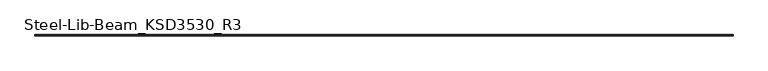
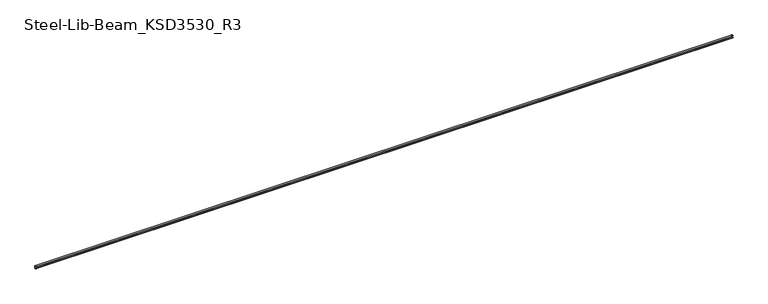
"""IFC4 building model written with IfcOpenShell, lengths in millimetres: beam geometry, Steel-Lib-Beam_KSD3530_R3 : BMS291_C-150×75x20x4.5."""

from ifc_helpers import new_model, si_unit, point, frame, frame_2d, origin, place, context, project, spatial, polyline, circle_curve, trimmed, segment, composite_curve, outline, extrude, source, transform, mapped, element, save


def steel_lib_beam_ksd3530_r3_56628b3c(model_context):
    return source(origin(), model_context, "Body", "SweptSolid", [
        extrude(outline(composite_curve([segment(trimmed(circle_curve(frame_2d((-41.0, 66.0)), 9.0), [point((-50.0, 66.0))], [point((-41.0, 75.0))], False, "CARTESIAN"), True, "CONTINUOUS"), segment(polyline([(-41.0, 75.0), (16.0, 75.0)]), True, "CONTINUOUS"), segment(trimmed(circle_curve(frame_2d((16.0, 66.0)), 9.0), [point((16.0, 75.0))], [point((25.0, 66.0))], False, "CARTESIAN"), True, "CONTINUOUS"), segment(polyline([(25.0, 66.0), (25.0, -66.0)]), True, "CONTINUOUS"), segment(trimmed(circle_curve(frame_2d((16.0, -66.0)), 9.0), [point((25.0, -66.0))], [point((16.0, -75.0))], False, "CARTESIAN"), True, "CONTINUOUS"), segment(polyline([(16.0, -75.0), (-41.0, -75.0)]), True, "CONTINUOUS"), segment(trimmed(circle_curve(frame_2d((-41.0, -66.0)), 9.0), [point((-41.0, -75.0))], [point((-50.0, -66.0))], False, "CARTESIAN"), True, "CONTINUOUS"), segment(polyline([(-50.0, -66.0), (-50.0, -55.0), (-45.5, -55.0), (-45.5, -66.0)]), True, "CONTINUOUS"), segment(trimmed(circle_curve(frame_2d((-41.0, -66.0)), 4.5), [point((-45.5, -66.0))], [point((-41.0, -70.5))], True, "CARTESIAN"), True, "CONTINUOUS"), segment(polyline([(-41.0, -70.5), (16.0, -70.5)]), True, "CONTINUOUS"), segment(trimmed(circle_curve(frame_2d((16.0, -66.0)), 4.5), [point((16.0, -70.5))], [point((20.5, -66.0))], True, "CARTESIAN"), True, "CONTINUOUS"), segment(polyline([(20.5, -66.0), (20.5, 66.0)]), True, "CONTINUOUS"), segment(trimmed(circle_curve(frame_2d((16.0, 66.0)), 4.5), [point((20.5, 66.0))], [point((16.0, 70.5))], True, "CARTESIAN"), True, "CONTINUOUS"), segment(polyline([(16.0, 70.5), (-41.0, 70.5)]), True, "CONTINUOUS"), segment(trimmed(circle_curve(frame_2d((-41.0, 66.0)), 4.5), [point((-41.0, 70.5))], [point((-45.5, 66.0))], True, "CARTESIAN"), True, "CONTINUOUS"), segment(polyline([(-45.5, 66.0), (-45.5, 55.0), (-50.0, 55.0), (-50.0, 66.0)]), True, "CONTINUOUS")], self_intersect=False)), frame((-20487.3, 0.0, 0.0), z_axis=(1.0, 0.0, 0.0), x_axis=(0.0, 1.0, 0.0)), (0.0, 0.0, 1.0), 40924.6),
    ])


if __name__ == "__main__":
    model = new_model("IFC4")
    model_context = context("Model", 3, world=origin())
    ifc_project = project(units=[si_unit("LENGTHUNIT", "METRE", prefix="MILLI")], contexts=[model_context])
    site = spatial("IfcSite", under=ifc_project)
    building = spatial("IfcBuilding", under=site)
    placement = place(None, origin())
    steel_lib_beam_ksd3530_r3_shape = steel_lib_beam_ksd3530_r3_56628b3c(model_context)
    element("IfcBeam", 1, ObjectType="Steel-Lib-Beam_KSD3530_R3 : BMS291_C-150×75x20x4.5", at=placement, inside=building, context=model_context, shape_type="MappedRepresentation", body=[
        mapped(steel_lib_beam_ksd3530_r3_shape, transform((0.0, 0.0, 0.0), x_axis=(1.0, 0.0, 0.0), y_axis=(0.0, 1.0, 0.0), z_axis=(0.0, 0.0, 1.0))),
    ])
    save(model, "model.ifc")

# Revit data of these elements
# Type "Steel-Lib-Beam_KSD3530_R3 : BMS291_C-150×75x20x4.5"
#   Keynote = "C-150×75x20x4.5"
#   SteelWeight = "Light"
#   x = 0.0250 m
#   t1 = 0.0090 m
#   t = 0.0045 m
#   Surface Area = 0.629834 m²/m
#   Section Area = 13.9688 cm²
#   Mass per Unit Length = 10.9655 kg/m
#   C = 0.0200 m
#   A = 0.0750 m
#   Length [instance default] = 1.5000 m
#   H = 0.1500 m
#   hec_material4 [instance default] = none
#   hec_material3 [instance default] = none
#   hec_material2 [instance default] = none
#   hec_material1 [instance default] = none
#   Structural Material [instance default] = Metal - Steel - Light Gauge
#   Assembly Code = ""
# Element 1 (IfcBeam, "Steel-Lib-Beam_KSD3530_R3 : BMS291_C-150×75x20x4.5")
#   Structural Material = none
# Materials
#   "Metal - Steel - Light Gauge": class "Metal", colour RGB 247 247 247, transparency 0
